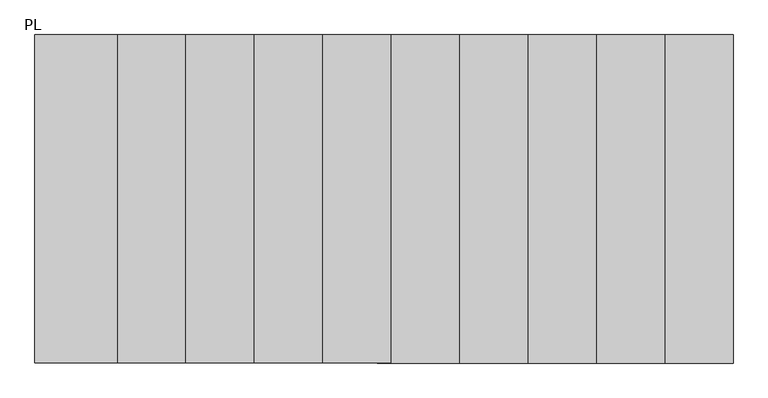
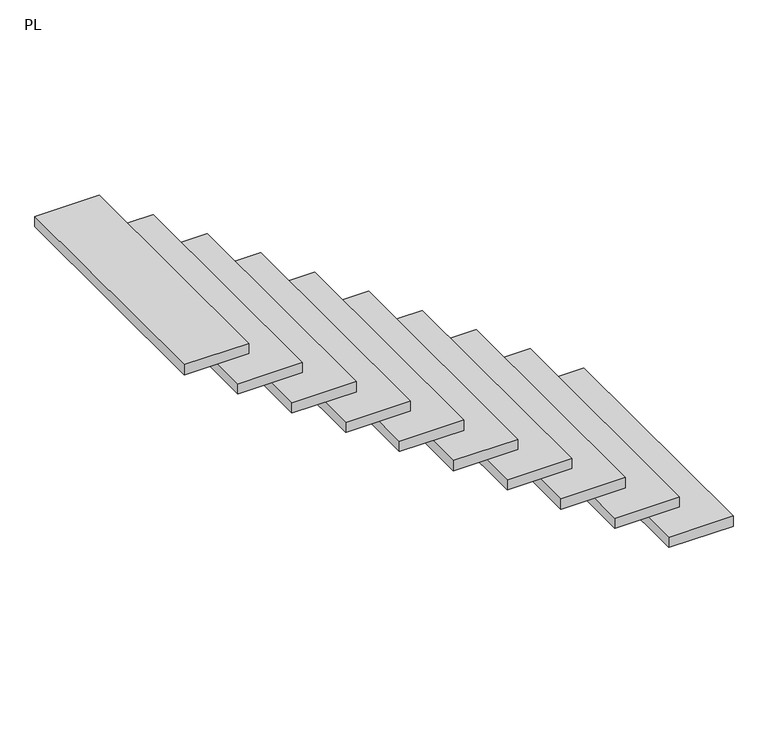
"""IFC4 building model written with IfcOpenShell, lengths in millimetres: stair flight geometry, PL."""

import ifcopenshell
import ifcopenshell.guid

model = None  # the IFC model being written
_history = None  # IfcOwnerHistory: only IFC2X3 demands one
_inside = {}  # id of a spatial element -> (the spatial element, [elements in it])
_under = {}  # id of a project, library or spatial element -> (it, [spatial elements below it])
_declared = {}  # id of a project -> (the project, [libraries it declares])
_typed = {}  # id of a type object -> (the type object, [elements of that type])
_made_of = {}  # id of a material, layer set ... -> (it, [elements and type objects made of it])


def new_model(schema):
    """Start an empty IFC model of exactly this schema.

    Asked for "IFC4X3", IfcOpenShell would pick the latest addendum, in which some entities
    have other attributes; the version numbers below select the first issue.
    IFC2X3 requires an IfcOwnerHistory on every rooted entity: one is made here for all.
    """
    global model, _history
    if schema == "IFC4X3":
        model = ifcopenshell.file(schema_version=(4, 3, 0, 0))
    else:
        model = ifcopenshell.file(schema=schema)
    _inside.clear()
    _under.clear()
    _declared.clear()
    _typed.clear()
    _made_of.clear()
    _history = None
    if model.schema == "IFC2X3":
        org = make("IfcOrganization", Name="unknown")
        user = make(
            "IfcPersonAndOrganization",
            ThePerson=make("IfcPerson", FamilyName="unknown"),
            TheOrganization=org,
        )
        app = make(
            "IfcApplication",
            ApplicationDeveloper=org,
            Version="unknown",
            ApplicationFullName="unknown",
            ApplicationIdentifier="unknown",
        )
        _history = make(
            "IfcOwnerHistory",
            OwningUser=user,
            OwningApplication=app,
            ChangeAction="ADDED",
            CreationDate=0,
        )
    return model


def make(cls, **values):
    """One entity of the class cls with the attributes given. An attribute that is None is left unset."""
    return model.create_entity(
        cls, **{name: value for name, value in values.items() if value is not None}
    )


def rooted(cls, **values):
    """An entity with a GlobalId (a new one), such as an element, a storey or a relation."""
    return make(cls, GlobalId=ifcopenshell.guid.new(), OwnerHistory=_history, **values)


def si_unit(unit_type, name, prefix=None):
    """IfcSIUnit, for example si_unit("LENGTHUNIT", "METRE", prefix="MILLI")."""
    return make("IfcSIUnit", UnitType=unit_type, Prefix=prefix, Name=name)


def assignment(units):
    """IfcUnitAssignment: the units of a project."""
    return None if units is None else make("IfcUnitAssignment", Units=units)


def point(xyz):
    """IfcCartesianPoint."""
    return None if xyz is None else make("IfcCartesianPoint", Coordinates=xyz)


def direction(xyz):
    """IfcDirection."""
    return None if xyz is None else make("IfcDirection", DirectionRatios=xyz)


def frame(location, z_axis=None, x_axis=None):
    """IfcAxis2Placement3D, a coordinate frame: its origin and axes. An axis left out is left unset."""
    return make(
        "IfcAxis2Placement3D",
        Location=point(location),
        Axis=direction(z_axis),
        RefDirection=direction(x_axis),
    )


def origin():
    """The frame at (0, 0, 0) with its axes left unset."""
    return frame((0.0, 0.0, 0.0))


def place(relative_to, where):
    """IfcLocalPlacement: puts the frame where relative to a parent placement (None: the world)."""
    return make(
        "IfcLocalPlacement", PlacementRelTo=relative_to, RelativePlacement=where
    )


def context(
    kind, dimensions, precision=None, world=None, true_north=None, identifier=None
):
    """IfcGeometricRepresentationContext, for example the 3D "Model" context."""
    return make(
        "IfcGeometricRepresentationContext",
        ContextIdentifier=identifier,
        ContextType=kind,
        CoordinateSpaceDimension=dimensions,
        Precision=precision,
        WorldCoordinateSystem=world,
        TrueNorth=true_north,
    )


def project(units=None, contexts=None):
    """IfcProject with its units and contexts."""
    return rooted(
        "IfcProject",
        Name="project",
        RepresentationContexts=contexts,
        UnitsInContext=assignment(units),
    )


def spatial(cls, under=None, at=None, **own):
    """A site, building, storey or space (cls), placed at a placement, below another one or the project."""
    s = rooted(cls, ObjectPlacement=at, **own)
    if under is not None:
        _under.setdefault(under.id(), (under, []))[1].append(s)
    return s


def polyline(points):
    """IfcPolyline through the points."""
    return make("IfcPolyline", Points=[point(p) for p in points])


def outline(outer, holes=None, kind="AREA"):
    """IfcArbitraryClosedProfileDef: a profile drawn as a closed curve; with holes, ...WithVoids."""
    if holes is None:
        return make("IfcArbitraryClosedProfileDef", ProfileType=kind, OuterCurve=outer)
    return make(
        "IfcArbitraryProfileDefWithVoids",
        ProfileType=kind,
        OuterCurve=outer,
        InnerCurves=holes,
    )


def extrude(swept, where, along, depth):
    """IfcExtrudedAreaSolid: the profile swept, set in the frame where, extruded along a direction by depth."""
    return make(
        "IfcExtrudedAreaSolid",
        SweptArea=swept,
        Position=where,
        ExtrudedDirection=direction(along),
        Depth=depth,
    )


def shape(context_of_items, identifier, shape_type, items):
    """IfcShapeRepresentation: the items that make up one representation, for example the "Body"."""
    return make(
        "IfcShapeRepresentation",
        ContextOfItems=context_of_items,
        RepresentationIdentifier=identifier,
        RepresentationType=shape_type,
        Items=items,
    )


def source(mapping_origin, context_of_items, identifier, shape_type, items):
    """IfcRepresentationMap: a shape defined once, which mapped items show again and again."""
    return make(
        "IfcRepresentationMap",
        MappingOrigin=mapping_origin,
        MappedRepresentation=shape(context_of_items, identifier, shape_type, items),
    )


def transform(
    local_origin,
    x_axis=None,
    y_axis=None,
    z_axis=None,
    scale=None,
    scale2=None,
    scale3=None,
    uniform=True,
):
    """IfcCartesianTransformationOperator3D, or its non-uniform kind. x_axis, y_axis, z_axis: its Axis1, 2, 3."""
    if uniform:
        return make(
            "IfcCartesianTransformationOperator3D",
            Axis1=direction(x_axis),
            Axis2=direction(y_axis),
            LocalOrigin=point(local_origin),
            Scale=scale,
            Axis3=direction(z_axis),
        )
    return make(
        "IfcCartesianTransformationOperator3DnonUniform",
        Axis1=direction(x_axis),
        Axis2=direction(y_axis),
        LocalOrigin=point(local_origin),
        Scale=scale,
        Axis3=direction(z_axis),
        Scale2=scale2,
        Scale3=scale3,
    )


def mapped(mapping_source, mapping_target):
    """IfcMappedItem: shows the shape of a source again, moved by a transform."""
    return make(
        "IfcMappedItem", MappingSource=mapping_source, MappingTarget=mapping_target
    )


def made_of(thing, what):
    """Note that an element or type object is made of a material, layer set ...; save() writes the relation."""
    if what is not None:
        _made_of.setdefault(what.id(), (what, []))[1].append(thing)
    return thing


def element(
    cls,
    number,
    at=None,
    inside=None,
    cuts=None,
    type_object=None,
    material=None,
    context=None,
    identifier="Body",
    shape_type=None,
    held_by="IfcProductDefinitionShape",
    body=None,
    shapes=None,
    **own,
):
    """One element of the class cls, such as IfcWall. Its Tag is "e" and its number.

    at: its placement. inside: the storey or other place that contains it. cuts: it is an
    opening in that element (IfcRelVoidsElement). A single representation is given by context,
    identifier, shape_type and body (its items); several are given by shapes. held_by: the class
    of the entity that holds the representations. save() writes the other relations.
    """
    e = rooted(cls, Tag="e%d" % number, ObjectPlacement=at, **own)
    if body is not None:
        shapes = [shape(context, identifier, shape_type, body)]
    if shapes is not None:
        e.Representation = make(held_by, Representations=shapes)
    if inside is not None:
        _inside.setdefault(inside.id(), (inside, []))[1].append(e)
    if cuts is not None:
        rooted(
            "IfcRelVoidsElement", RelatingBuildingElement=cuts, RelatedOpeningElement=e
        )
    if type_object is not None:
        _typed.setdefault(type_object.id(), (type_object, []))[1].append(e)
    return made_of(e, material)


def aggregate(whole, parts):
    """IfcRelAggregates: a whole, such as a stair, and the parts it consists of."""
    return rooted("IfcRelAggregates", RelatingObject=whole, RelatedObjects=parts)


def save(model, path):
    """Write the relations noted so far, then the file.

    IfcRelAggregates (storeys below a building ...), IfcRelContainedInSpatialStructure (elements
    in a storey), IfcRelDefinesByType, IfcRelAssociatesMaterial and IfcRelDeclares: one each for
    every whole, place, type object, material and project.
    """
    for whole, parts in _under.values():
        aggregate(whole, parts)
    for where, things in _inside.values():
        rooted(
            "IfcRelContainedInSpatialStructure",
            RelatedElements=things,
            RelatingStructure=where,
        )
    for kind, things in _typed.values():
        rooted("IfcRelDefinesByType", RelatedObjects=things, RelatingType=kind)
    for what, things in _made_of.values():
        rooted("IfcRelAssociatesMaterial", RelatedObjects=things, RelatingMaterial=what)
    for by, libraries in _declared.values():
        rooted("IfcRelDeclares", RelatingContext=by, RelatedDefinitions=libraries)
    model.write(path)


def pl_11391cdb(model_context):
    return source(origin(), model_context, "Body", "SweptSolid", [
        extrude(outline(polyline([(6009.5374538, 38624.5208589), (6309.5374538, 38624.5208589), (6309.5374538, 37424.5208589), (6009.5374538, 37424.5208589), (6009.5374538, 38624.5208589)])), frame((0.0, 0.0, 731.7901873), z_axis=(0.0, 0.0, 1.0), x_axis=(1.0, 0.0, 0.0)), (0.0, 0.0, 1.0), 50.0),
        extrude(outline(polyline([(5759.5374538, 38624.5208589), (6059.5374538, 38624.5208589), (6059.5374538, 37424.5208589), (5759.5374538, 37424.5208589), (5759.5374538, 38624.5208589)])), frame((0.0, 0.0, 913.6083692), z_axis=(0.0, 0.0, 1.0), x_axis=(1.0, 0.0, 0.0)), (0.0, 0.0, 1.0), 50.0),
        extrude(outline(polyline([(5509.5374538, 38624.5208589), (5809.5374538, 38624.5208589), (5809.5374538, 37424.5208589), (5509.5374538, 37424.5208589), (5509.5374538, 38624.5208589)])), frame((0.0, 0.0, 1095.426551), z_axis=(0.0, 0.0, 1.0), x_axis=(1.0, 0.0, 0.0)), (0.0, 0.0, 1.0), 50.0),
        extrude(outline(polyline([(5259.5374538, 38624.5208589), (5559.5374538, 38624.5208589), (5559.5374538, 37424.5208589), (5259.5374538, 37424.5208589), (5259.5374538, 38624.5208589)])), frame((0.0, 0.0, 1277.2447328), z_axis=(0.0, 0.0, 1.0), x_axis=(1.0, 0.0, 0.0)), (0.0, 0.0, 1.0), 50.0),
        extrude(outline(polyline([(5009.5374538, 38624.5208589), (5309.5374538, 38624.5208589), (5309.5374538, 37424.5208589), (5009.5374538, 37424.5208589), (5009.5374538, 38624.5208589)])), frame((0.0, 0.0, 1459.0629146), z_axis=(0.0, 0.0, 1.0), x_axis=(1.0, 0.0, 0.0)), (0.0, 0.0, 1.0), 50.0),
        extrude(outline(polyline([(4759.5374538, 38624.5208589), (5059.5374538, 38624.5208589), (5059.5374538, 37424.5208589), (4759.5374538, 37424.5208589), (4759.5374538, 38624.5208589)])), frame((0.0, 0.0, 1640.8810964), z_axis=(0.0, 0.0, 1.0), x_axis=(1.0, 0.0, 0.0)), (0.0, 0.0, 1.0), 50.0),
        extrude(outline(polyline([(4509.5374538, 38624.5208589), (4809.5374538, 38624.5208589), (4809.5374538, 37424.5208589), (4509.5374538, 37424.5208589), (4509.5374538, 38624.5208589)])), frame((0.0, 0.0, 1822.6992783), z_axis=(0.0, 0.0, 1.0), x_axis=(1.0, 0.0, 0.0)), (0.0, 0.0, 1.0), 50.0),
        extrude(outline(polyline([(4259.5374538, 38624.5208589), (4559.5374538, 38624.5208589), (4559.5374538, 37424.5208589), (4259.5374538, 37424.5208589), (4259.5374538, 38624.5208589)])), frame((0.0, 0.0, 2004.5174601), z_axis=(0.0, 0.0, 1.0), x_axis=(1.0, 0.0, 0.0)), (0.0, 0.0, 1.0), 50.0),
        extrude(outline(polyline([(4009.5374538, 38624.5208589), (4309.5374538, 38624.5208589), (4309.5374538, 37424.5208589), (4009.5374538, 37424.5208589), (4009.5374538, 38624.5208589)])), frame((0.0, 0.0, 2186.3356419), z_axis=(0.0, 0.0, 1.0), x_axis=(1.0, 0.0, 0.0)), (0.0, 0.0, 1.0), 50.0),
        extrude(outline(polyline([(3759.5374538, 38624.5208589), (4059.5374538, 38624.5208589), (4059.5374538, 37424.5208589), (3759.5374538, 37424.5208589), (3759.5374538, 38624.5208589)])), frame((0.0, 0.0, 2368.1538237), z_axis=(0.0, 0.0, 1.0), x_axis=(1.0, 0.0, 0.0)), (0.0, 0.0, 1.0), 50.0),
    ])


if __name__ == "__main__":
    model = new_model("IFC4")
    model_context = context("Model", 3, world=origin())
    ifc_project = project(units=[si_unit("LENGTHUNIT", "METRE", prefix="MILLI")], contexts=[model_context])
    site = spatial("IfcSite", under=ifc_project)
    building = spatial("IfcBuilding", under=site)
    placement = place(None, origin())
    pl_shape = pl_11391cdb(model_context)
    element("IfcStairFlight", 1, ObjectType="PL", at=placement, inside=building, context=model_context, shape_type="MappedRepresentation", body=[
        mapped(pl_shape, transform((0.0, 0.0, 0.0), x_axis=(1.0, 0.0, 0.0), y_axis=(0.0, 1.0, 0.0), z_axis=(0.0, 0.0, 1.0))),
    ])
    save(model, "model.ifc")
